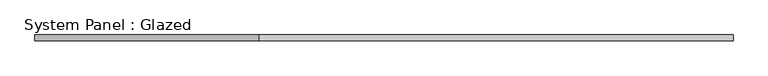
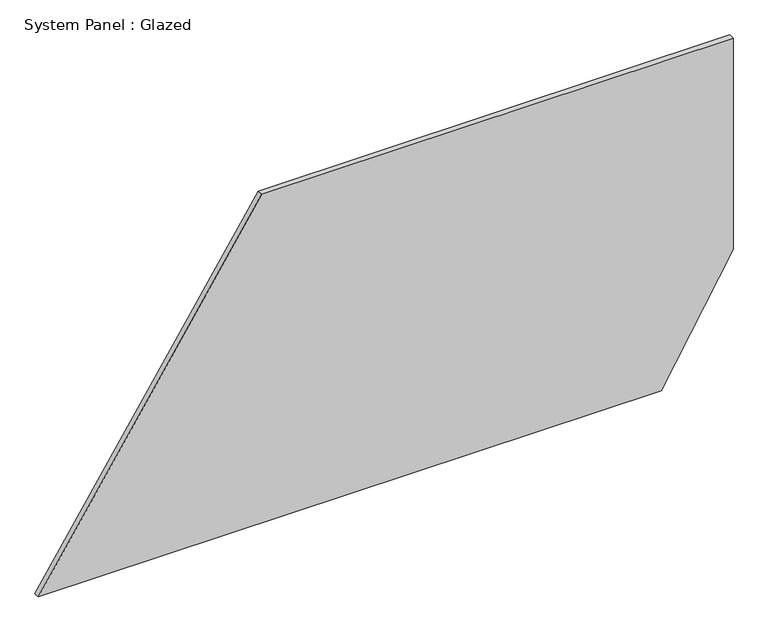
"""IFC4 building model written with IfcOpenShell, lengths in millimetres: plate geometry, System Panel : Glazed."""

from ifc_helpers import new_model, si_unit, frame, origin, place, context, project, spatial, polyline, outline, extrude, source, transform, mapped, element, save


def system_panel_glazed_b5708c6c(model_context):
    return source(origin(), model_context, "Body", "SweptSolid", [
        extrude(outline(polyline([(0.0, -1500.0000002), (0.0, 1190.2722385), (536.082289, 1500.0000002), (1500.0, 1500.0000002), (1500.0, -535.7030249), (0.0, -1500.0000002)])), frame((0.0, 24.5, 0.0), z_axis=(0.0, 1.0, 0.0), x_axis=(0.0, 0.0, 1.0)), (0.0, 0.0, 1.0), 25.0),
    ])


if __name__ == "__main__":
    model = new_model("IFC4")
    model_context = context("Model", 3, world=origin())
    ifc_project = project(units=[si_unit("LENGTHUNIT", "METRE", prefix="MILLI")], contexts=[model_context])
    site = spatial("IfcSite", under=ifc_project)
    building = spatial("IfcBuilding", under=site)
    placement = place(None, origin())
    system_panel_glazed_shape = system_panel_glazed_b5708c6c(model_context)
    element("IfcPlate", 1, ObjectType="System Panel : Glazed", at=placement, inside=building, context=model_context, shape_type="MappedRepresentation", body=[
        mapped(system_panel_glazed_shape, transform((0.0, 0.0, 0.0), x_axis=(1.0, 0.0, 0.0), y_axis=(0.0, 1.0, 0.0), z_axis=(0.0, 0.0, 1.0))),
    ])
    save(model, "model.ifc")

# Revit data of these elements
# Type "System Panel : Glazed"
#   Construction Type Id = "GSP4R"
#   Analytic Construction = "1/8 in Pilkington single glazing"
#   Visual Light Transmittance = 0.9
#   Solar Heat Gain Coefficient = 0.86
#   Heat Transfer Coefficient (U) = 6.7069 W/(m²·K)
#   Define Thermal Properties by = 1
# Element 1 (IfcPlate, "System Panel : Glazed")
#   Materials on its faces: "Glass"
# Materials
#   "Glass": class "Glass", colour RGB 0 128 192, transparency 0.9, Description = "Soda Lime Glass", Cost = 0
